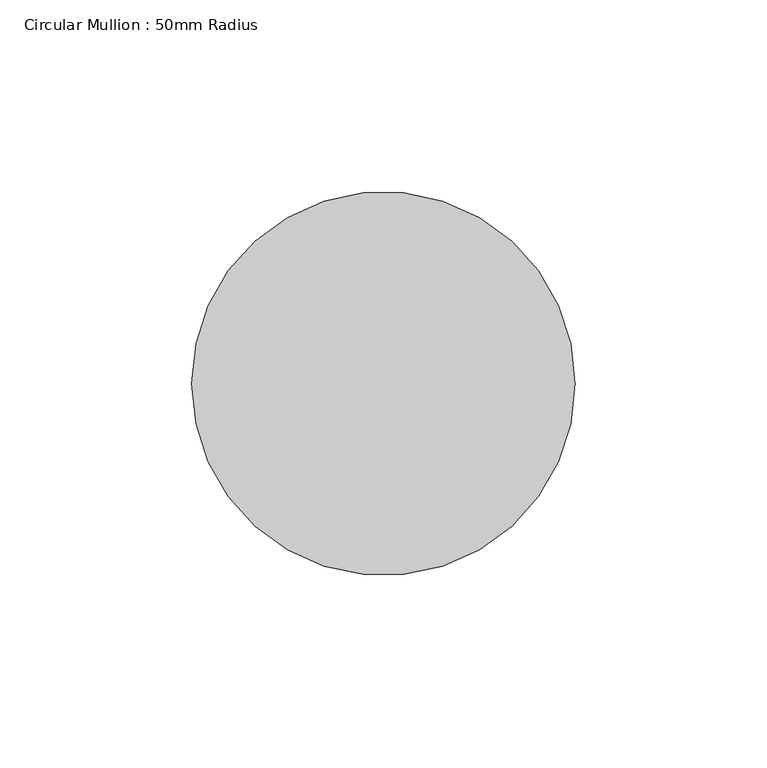
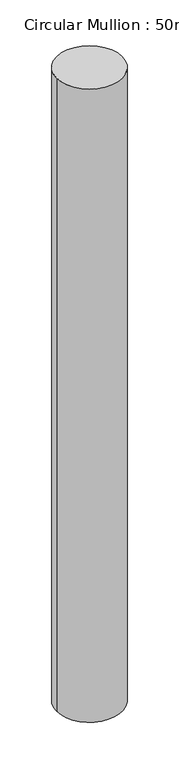
"""IFC4 building model written with IfcOpenShell, lengths in millimetres: member geometry, Circular Mullion : 50mm Radius."""

from ifc_helpers import new_model, si_unit, point, frame, origin, origin_2d, place, context, project, spatial, circle_curve, trimmed, segment, composite_curve, outline, extrude, source, transform, mapped, element, save


def circular_mullion_50mm_radius_d9d6dba5(model_context):
    return source(origin(), model_context, "Body", "SweptSolid", [
        extrude(outline(composite_curve([segment(trimmed(circle_curve(origin_2d(), 50.0), [point((50.0, 0.0))], [point((-50.0, 0.0))], False, "CARTESIAN"), True, "CONTINUOUS"), segment(trimmed(circle_curve(origin_2d(), 50.0), [point((-50.0, 0.0))], [point((50.0, 0.0))], False, "CARTESIAN"), True, "CONTINUOUS")], self_intersect=False)), frame((0.0, 0.0, -1022.3928664), z_axis=(0.0, 0.0, 1.0), x_axis=(1.0, 0.0, 0.0)), (0.0, 0.0, 1.0), 1022.3928664),
    ])


if __name__ == "__main__":
    model = new_model("IFC4")
    model_context = context("Model", 3, world=origin())
    ifc_project = project(units=[si_unit("LENGTHUNIT", "METRE", prefix="MILLI")], contexts=[model_context])
    site = spatial("IfcSite", under=ifc_project)
    building = spatial("IfcBuilding", under=site)
    placement = place(None, origin())
    circular_mullion_50mm_radius_shape = circular_mullion_50mm_radius_d9d6dba5(model_context)
    element("IfcMember", 1, ObjectType="Circular Mullion : 50mm Radius", at=placement, inside=building, context=model_context, shape_type="MappedRepresentation", body=[
        mapped(circular_mullion_50mm_radius_shape, transform((0.0, 0.0, 0.0), x_axis=(1.0, 0.0, 0.0), y_axis=(0.0, 1.0, 0.0), z_axis=(0.0, 0.0, 1.0))),
    ])
    save(model, "model.ifc")

# Revit data of these elements
# Type "Circular Mullion : 50mm Radius"
#   built-in parameter 1007350 = 0.164042 (stored number, unit not read)
# Element 1 (IfcMember, "Circular Mullion : 50mm Radius")
#   Materials on its faces: "Aluminium"
# Materials
#   "Aluminium": class "Metal", colour RGB 247 247 247, transparency 0, Description = "Aluminium 6061", Cost = 0
